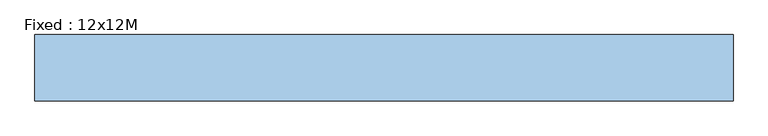
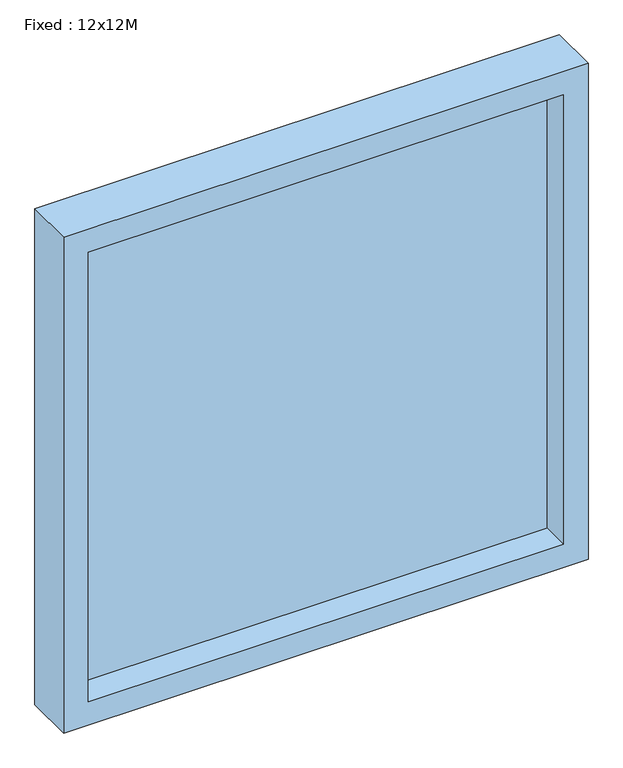
"""IFC4 building model written with IfcOpenShell, lengths in millimetres: window geometry, Fixed : 12x12M."""

from ifc_helpers import new_model, si_unit, frame, origin, place, context, project, spatial, polyline, outline, extrude, source, transform, mapped, element, save


def fixed_12x12m_54af5089(model_context):
    return source(origin(), model_context, "Body", "SweptSolid", [
        extrude(outline(polyline([(2012.0, 606.0), (2012.0, -606.0), (800.0, -606.0), (800.0, 606.0), (2012.0, 606.0)]), holes=[polyline([(857.0, 549.0), (857.0, -549.0), (1955.0, -549.0), (1955.0, 549.0), (857.0, 549.0)])]), frame((0.0, 69.0, 0.0), z_axis=(0.0, 1.0, 0.0), x_axis=(0.0, 0.0, 1.0)), (0.0, 0.0, 1.0), 115.0),
        extrude(outline(polyline([(-549.0, 162.0), (549.0, 162.0), (549.0, 134.0), (-549.0, 134.0), (-549.0, 162.0)])), frame((0.0, 0.0, 857.0), z_axis=(0.0, 0.0, 1.0), x_axis=(1.0, 0.0, 0.0)), (0.0, 0.0, 1.0), 1098.0),
    ])


if __name__ == "__main__":
    model = new_model("IFC4")
    model_context = context("Model", 3, world=origin())
    ifc_project = project(units=[si_unit("LENGTHUNIT", "METRE", prefix="MILLI")], contexts=[model_context])
    site = spatial("IfcSite", under=ifc_project)
    building = spatial("IfcBuilding", under=site)
    placement = place(None, origin())
    fixed_12x12m_shape = fixed_12x12m_54af5089(model_context)
    element("IfcWindow", 1, ObjectType="Fixed : 12x12M", at=placement, inside=building, context=model_context, shape_type="MappedRepresentation", body=[
        mapped(fixed_12x12m_shape, transform((0.0, 0.0, 0.0), x_axis=(1.0, 0.0, 0.0), y_axis=(0.0, 1.0, 0.0), z_axis=(0.0, 0.0, 1.0))),
    ])
    save(model, "model.ifc")

# Revit data of these elements
# Type "Fixed : 12x12M"
#   Type Mark = "55"
#   Creator Organization [instance default] = "© Danish Educational Content"
#   Creator Name [instance default] = "© Erik Falck Jørgensen"
#   Creator Build [instance default] = "2017.0801.0"
#   Analytic Construction = "<None>"
#   length#5 = -22 mm
#   length#4 = -50 mm
#   length#3 = 100 mm
#   length#2 = 57 mm
#   length#1 = 0 mm
#   Seal Width = 12 mm
#   Rough Width = 1212 mm
#   Rough Height = 1212 mm
#   Rebate Depth = 50 mm
#   Height = 1188 mm
#   Glass Thickness = 28 mm
#   Exterior Direction [instance default] = 0.00°
#   Default Sill Height = 800 mm
#   Width = 1188 mm
#   Case Width = 45 mm
#   Case Depth = 115 mm
#   Sealing = no
#   Wall Closure = 1
#   Above Cutplane [instance default] = no
#   Wall Surface = none
#   Sill Plate = none
#   Glass = none
#   Embrasure = none
#   Case/Transom = none
#   Assembly Code = ""
# Element 1 (IfcWindow, "Fixed : 12x12M")
#   Materials on its faces: "Default Frame/Mullion (Interior/Exterior)", "Glass"
# Materials
#   "Default Frame/Mullion (Interior/Exterior)": class "Generic", colour RGB 205 205 205, transparency 0, Description = "Udefineret karm/ramme materiale", Cost = 0
#   "Glass": class "Glass", colour RGB 180 200 255, transparency 0.75, Description = "Generisk glas", Cost = 0
